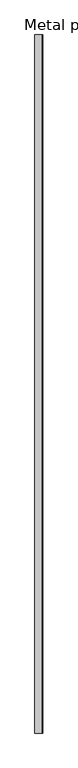
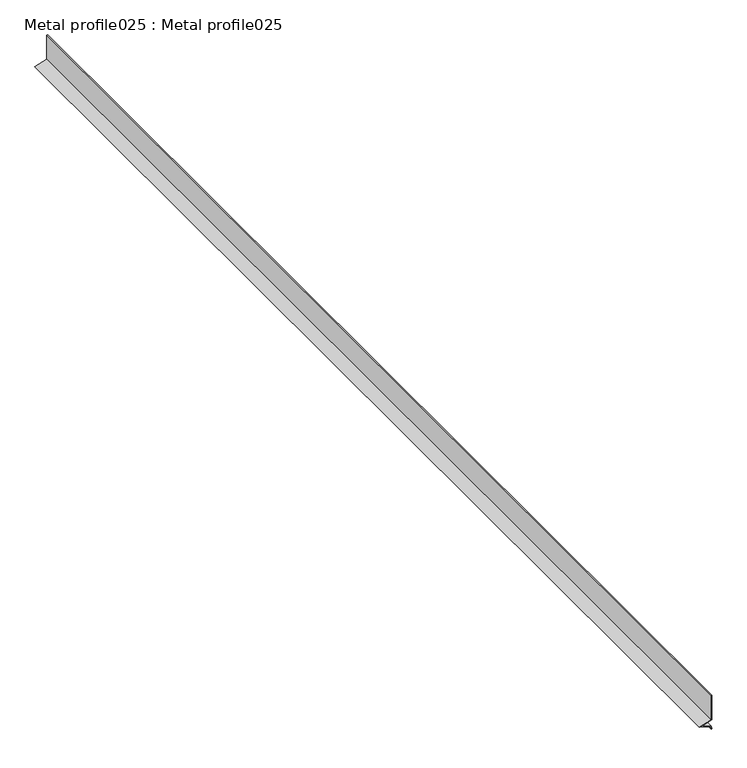
"""IFC4 building model written with IfcOpenShell, lengths in millimetres: proxy geometry, Metal profile025 : Metal profile025."""

import ifcopenshell
import ifcopenshell.guid

model = None  # the IFC model being written
_history = None  # IfcOwnerHistory: only IFC2X3 demands one
_inside = {}  # id of a spatial element -> (the spatial element, [elements in it])
_under = {}  # id of a project, library or spatial element -> (it, [spatial elements below it])
_declared = {}  # id of a project -> (the project, [libraries it declares])
_typed = {}  # id of a type object -> (the type object, [elements of that type])
_made_of = {}  # id of a material, layer set ... -> (it, [elements and type objects made of it])


def new_model(schema):
    """Start an empty IFC model of exactly this schema.

    Asked for "IFC4X3", IfcOpenShell would pick the latest addendum, in which some entities
    have other attributes; the version numbers below select the first issue.
    IFC2X3 requires an IfcOwnerHistory on every rooted entity: one is made here for all.
    """
    global model, _history
    if schema == "IFC4X3":
        model = ifcopenshell.file(schema_version=(4, 3, 0, 0))
    else:
        model = ifcopenshell.file(schema=schema)
    _inside.clear()
    _under.clear()
    _declared.clear()
    _typed.clear()
    _made_of.clear()
    _history = None
    if model.schema == "IFC2X3":
        org = make("IfcOrganization", Name="unknown")
        user = make(
            "IfcPersonAndOrganization",
            ThePerson=make("IfcPerson", FamilyName="unknown"),
            TheOrganization=org,
        )
        app = make(
            "IfcApplication",
            ApplicationDeveloper=org,
            Version="unknown",
            ApplicationFullName="unknown",
            ApplicationIdentifier="unknown",
        )
        _history = make(
            "IfcOwnerHistory",
            OwningUser=user,
            OwningApplication=app,
            ChangeAction="ADDED",
            CreationDate=0,
        )
    return model


def make(cls, **values):
    """One entity of the class cls with the attributes given. An attribute that is None is left unset."""
    return model.create_entity(
        cls, **{name: value for name, value in values.items() if value is not None}
    )


def rooted(cls, **values):
    """An entity with a GlobalId (a new one), such as an element, a storey or a relation."""
    return make(cls, GlobalId=ifcopenshell.guid.new(), OwnerHistory=_history, **values)


def si_unit(unit_type, name, prefix=None):
    """IfcSIUnit, for example si_unit("LENGTHUNIT", "METRE", prefix="MILLI")."""
    return make("IfcSIUnit", UnitType=unit_type, Prefix=prefix, Name=name)


def assignment(units):
    """IfcUnitAssignment: the units of a project."""
    return None if units is None else make("IfcUnitAssignment", Units=units)


def point(xyz):
    """IfcCartesianPoint."""
    return None if xyz is None else make("IfcCartesianPoint", Coordinates=xyz)


def direction(xyz):
    """IfcDirection."""
    return None if xyz is None else make("IfcDirection", DirectionRatios=xyz)


def frame(location, z_axis=None, x_axis=None):
    """IfcAxis2Placement3D, a coordinate frame: its origin and axes. An axis left out is left unset."""
    return make(
        "IfcAxis2Placement3D",
        Location=point(location),
        Axis=direction(z_axis),
        RefDirection=direction(x_axis),
    )


def origin():
    """The frame at (0, 0, 0) with its axes left unset."""
    return frame((0.0, 0.0, 0.0))


def place(relative_to, where):
    """IfcLocalPlacement: puts the frame where relative to a parent placement (None: the world)."""
    return make(
        "IfcLocalPlacement", PlacementRelTo=relative_to, RelativePlacement=where
    )


def context(
    kind, dimensions, precision=None, world=None, true_north=None, identifier=None
):
    """IfcGeometricRepresentationContext, for example the 3D "Model" context."""
    return make(
        "IfcGeometricRepresentationContext",
        ContextIdentifier=identifier,
        ContextType=kind,
        CoordinateSpaceDimension=dimensions,
        Precision=precision,
        WorldCoordinateSystem=world,
        TrueNorth=true_north,
    )


def project(units=None, contexts=None):
    """IfcProject with its units and contexts."""
    return rooted(
        "IfcProject",
        Name="project",
        RepresentationContexts=contexts,
        UnitsInContext=assignment(units),
    )


def spatial(cls, under=None, at=None, **own):
    """A site, building, storey or space (cls), placed at a placement, below another one or the project."""
    s = rooted(cls, ObjectPlacement=at, **own)
    if under is not None:
        _under.setdefault(under.id(), (under, []))[1].append(s)
    return s


def polyline(points):
    """IfcPolyline through the points."""
    return make("IfcPolyline", Points=[point(p) for p in points])


def outline(outer, holes=None, kind="AREA"):
    """IfcArbitraryClosedProfileDef: a profile drawn as a closed curve; with holes, ...WithVoids."""
    if holes is None:
        return make("IfcArbitraryClosedProfileDef", ProfileType=kind, OuterCurve=outer)
    return make(
        "IfcArbitraryProfileDefWithVoids",
        ProfileType=kind,
        OuterCurve=outer,
        InnerCurves=holes,
    )


def extrude(swept, where, along, depth):
    """IfcExtrudedAreaSolid: the profile swept, set in the frame where, extruded along a direction by depth."""
    return make(
        "IfcExtrudedAreaSolid",
        SweptArea=swept,
        Position=where,
        ExtrudedDirection=direction(along),
        Depth=depth,
    )


def shape(context_of_items, identifier, shape_type, items):
    """IfcShapeRepresentation: the items that make up one representation, for example the "Body"."""
    return make(
        "IfcShapeRepresentation",
        ContextOfItems=context_of_items,
        RepresentationIdentifier=identifier,
        RepresentationType=shape_type,
        Items=items,
    )


def source(mapping_origin, context_of_items, identifier, shape_type, items):
    """IfcRepresentationMap: a shape defined once, which mapped items show again and again."""
    return make(
        "IfcRepresentationMap",
        MappingOrigin=mapping_origin,
        MappedRepresentation=shape(context_of_items, identifier, shape_type, items),
    )


def transform(
    local_origin,
    x_axis=None,
    y_axis=None,
    z_axis=None,
    scale=None,
    scale2=None,
    scale3=None,
    uniform=True,
):
    """IfcCartesianTransformationOperator3D, or its non-uniform kind. x_axis, y_axis, z_axis: its Axis1, 2, 3."""
    if uniform:
        return make(
            "IfcCartesianTransformationOperator3D",
            Axis1=direction(x_axis),
            Axis2=direction(y_axis),
            LocalOrigin=point(local_origin),
            Scale=scale,
            Axis3=direction(z_axis),
        )
    return make(
        "IfcCartesianTransformationOperator3DnonUniform",
        Axis1=direction(x_axis),
        Axis2=direction(y_axis),
        LocalOrigin=point(local_origin),
        Scale=scale,
        Axis3=direction(z_axis),
        Scale2=scale2,
        Scale3=scale3,
    )


def mapped(mapping_source, mapping_target):
    """IfcMappedItem: shows the shape of a source again, moved by a transform."""
    return make(
        "IfcMappedItem", MappingSource=mapping_source, MappingTarget=mapping_target
    )


def made_of(thing, what):
    """Note that an element or type object is made of a material, layer set ...; save() writes the relation."""
    if what is not None:
        _made_of.setdefault(what.id(), (what, []))[1].append(thing)
    return thing


def element(
    cls,
    number,
    at=None,
    inside=None,
    cuts=None,
    type_object=None,
    material=None,
    context=None,
    identifier="Body",
    shape_type=None,
    held_by="IfcProductDefinitionShape",
    body=None,
    shapes=None,
    **own,
):
    """One element of the class cls, such as IfcWall. Its Tag is "e" and its number.

    at: its placement. inside: the storey or other place that contains it. cuts: it is an
    opening in that element (IfcRelVoidsElement). A single representation is given by context,
    identifier, shape_type and body (its items); several are given by shapes. held_by: the class
    of the entity that holds the representations. save() writes the other relations.
    """
    e = rooted(cls, Tag="e%d" % number, ObjectPlacement=at, **own)
    if body is not None:
        shapes = [shape(context, identifier, shape_type, body)]
    if shapes is not None:
        e.Representation = make(held_by, Representations=shapes)
    if inside is not None:
        _inside.setdefault(inside.id(), (inside, []))[1].append(e)
    if cuts is not None:
        rooted(
            "IfcRelVoidsElement", RelatingBuildingElement=cuts, RelatedOpeningElement=e
        )
    if type_object is not None:
        _typed.setdefault(type_object.id(), (type_object, []))[1].append(e)
    return made_of(e, material)


def aggregate(whole, parts):
    """IfcRelAggregates: a whole, such as a stair, and the parts it consists of."""
    return rooted("IfcRelAggregates", RelatingObject=whole, RelatedObjects=parts)


def save(model, path):
    """Write the relations noted so far, then the file.

    IfcRelAggregates (storeys below a building ...), IfcRelContainedInSpatialStructure (elements
    in a storey), IfcRelDefinesByType, IfcRelAssociatesMaterial and IfcRelDeclares: one each for
    every whole, place, type object, material and project.
    """
    for whole, parts in _under.values():
        aggregate(whole, parts)
    for where, things in _inside.values():
        rooted(
            "IfcRelContainedInSpatialStructure",
            RelatedElements=things,
            RelatingStructure=where,
        )
    for kind, things in _typed.values():
        rooted("IfcRelDefinesByType", RelatedObjects=things, RelatingType=kind)
    for what, things in _made_of.values():
        rooted("IfcRelAssociatesMaterial", RelatedObjects=things, RelatingMaterial=what)
    for by, libraries in _declared.values():
        rooted("IfcRelDeclares", RelatingContext=by, RelatedDefinitions=libraries)
    model.write(path)


def metal_profile025_metal_profile025_e0bbe71d(model_context):
    return source(origin(), model_context, "Body", "SweptSolid", [
        extrude(outline(polyline([(33322.0337932, -9678.6315139), (33327.1485436, -9679.594709), (33332.6487015, -9696.7063117), (33338.458458, -9678.6315139), (33383.4487015, -9678.6315139), (33383.4487015, -9679.9015139), (33339.3842373, -9679.9015139), (33332.6487015, -9700.8565139), (33326.1707534, -9680.7028974), (33321.7987616, -9679.8795765), (33322.0337932, -9678.6315139)])), frame((0.0, 7982.1529359, 0.0), z_axis=(0.0, 1.0, 0.0), x_axis=(0.0, 0.0, 1.0)), (0.0, 0.0, 1.0), 2000.0),
    ])


if __name__ == "__main__":
    model = new_model("IFC4")
    model_context = context("Model", 3, world=origin())
    ifc_project = project(units=[si_unit("LENGTHUNIT", "METRE", prefix="MILLI")], contexts=[model_context])
    site = spatial("IfcSite", under=ifc_project)
    building = spatial("IfcBuilding", under=site)
    placement = place(None, origin())
    metal_profile025_metal_profile025_shape = metal_profile025_metal_profile025_e0bbe71d(model_context)
    element("IfcBuildingElementProxy", 1, Name="Metal profile025 : Metal profile025", ObjectType="Metal profile025 : Metal profile025", at=placement, inside=building, context=model_context, shape_type="MappedRepresentation", body=[
        mapped(metal_profile025_metal_profile025_shape, transform((0.0, 0.0, 0.0), x_axis=(1.0, 0.0, 0.0), y_axis=(0.0, 1.0, 0.0), z_axis=(0.0, 0.0, 1.0))),
    ])
    save(model, "model.ifc")

# Revit data of these elements
# Type "Metal profile025 : Metal profile025"
#   NameOverride = "Metal profile025"
# Element 1 (IfcBuildingElementProxy, "Metal profile025 : Metal profile025")
#   Materials on its faces: "16 GA. COPPER WEEP SCREED W/ MIN 3 1/2\" ATTACHMENT FLANGE - LAP UNDERLAYMENT OVER WEED SCREED"
# Materials
#   "16 GA. COPPER WEEP SCREED W/ MIN 3 1/2\" ATTACHMENT FLANGE - LAP UNDERLAYMENT OVER WEED SCREED": class "Unassigned", colour RGB 255 237 20, transparency 0
